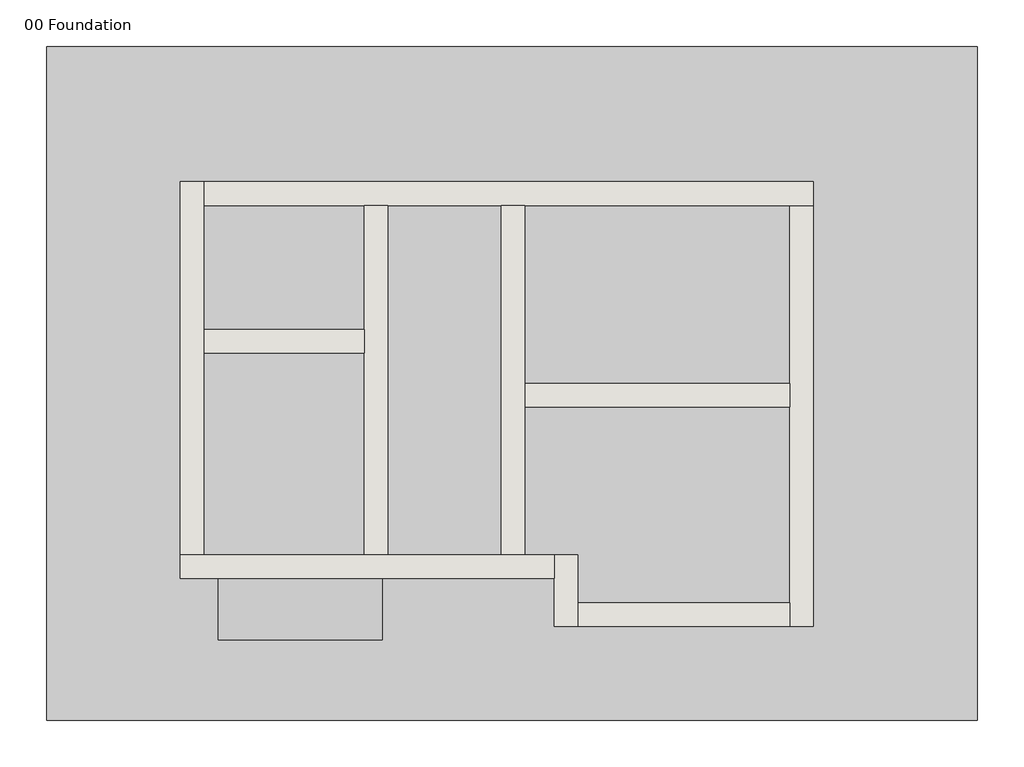
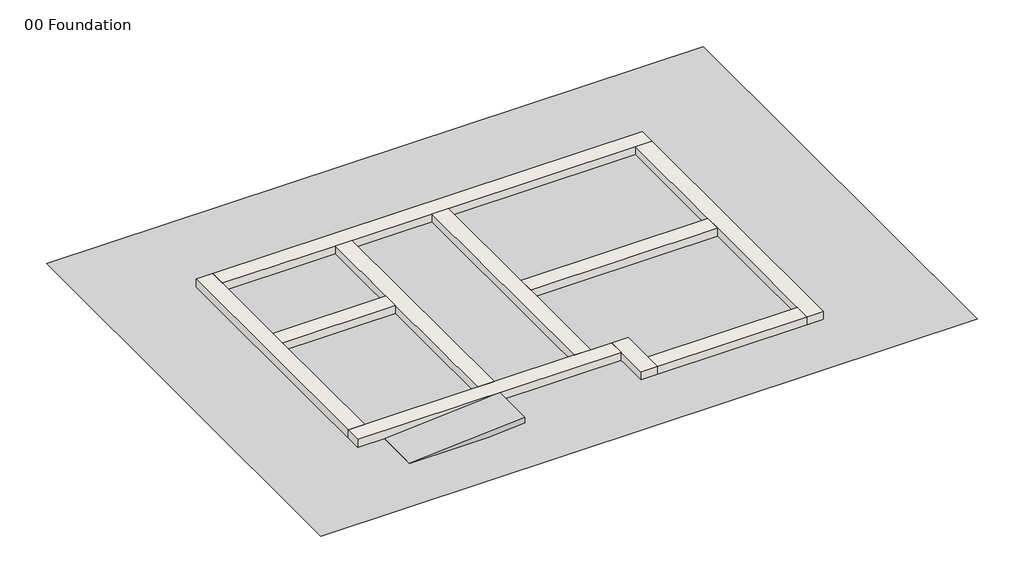
# One storey: 10 footings, 10 walls, 1 proxy, 1 ramp.
"""IFC4 building model written with IfcOpenShell, lengths in millimetres."""

import ifcopenshell
import ifcopenshell.guid

model = None  # the IFC model being written
_history = None  # IfcOwnerHistory: only IFC2X3 demands one
_inside = {}  # id of a spatial element -> (the spatial element, [elements in it])
_under = {}  # id of a project, library or spatial element -> (it, [spatial elements below it])
_declared = {}  # id of a project -> (the project, [libraries it declares])
_typed = {}  # id of a type object -> (the type object, [elements of that type])
_made_of = {}  # id of a material, layer set ... -> (it, [elements and type objects made of it])


def new_model(schema):
    """Start an empty IFC model of exactly this schema.

    Asked for "IFC4X3", IfcOpenShell would pick the latest addendum, in which some entities
    have other attributes; the version numbers below select the first issue.
    IFC2X3 requires an IfcOwnerHistory on every rooted entity: one is made here for all.
    """
    global model, _history
    if schema == "IFC4X3":
        model = ifcopenshell.file(schema_version=(4, 3, 0, 0))
    else:
        model = ifcopenshell.file(schema=schema)
    _inside.clear()
    _under.clear()
    _declared.clear()
    _typed.clear()
    _made_of.clear()
    _history = None
    if model.schema == "IFC2X3":
        org = make("IfcOrganization", Name="unknown")
        user = make(
            "IfcPersonAndOrganization",
            ThePerson=make("IfcPerson", FamilyName="unknown"),
            TheOrganization=org,
        )
        app = make(
            "IfcApplication",
            ApplicationDeveloper=org,
            Version="unknown",
            ApplicationFullName="unknown",
            ApplicationIdentifier="unknown",
        )
        _history = make(
            "IfcOwnerHistory",
            OwningUser=user,
            OwningApplication=app,
            ChangeAction="ADDED",
            CreationDate=0,
        )
    return model


def make(cls, **values):
    """One entity of the class cls with the attributes given. An attribute that is None is left unset."""
    return model.create_entity(
        cls, **{name: value for name, value in values.items() if value is not None}
    )


def rooted(cls, **values):
    """An entity with a GlobalId (a new one), such as an element, a storey or a relation."""
    return make(cls, GlobalId=ifcopenshell.guid.new(), OwnerHistory=_history, **values)


def si_unit(unit_type, name, prefix=None):
    """IfcSIUnit, for example si_unit("LENGTHUNIT", "METRE", prefix="MILLI")."""
    return make("IfcSIUnit", UnitType=unit_type, Prefix=prefix, Name=name)


def assignment(units):
    """IfcUnitAssignment: the units of a project."""
    return None if units is None else make("IfcUnitAssignment", Units=units)


def point(xyz):
    """IfcCartesianPoint."""
    return None if xyz is None else make("IfcCartesianPoint", Coordinates=xyz)


def direction(xyz):
    """IfcDirection."""
    return None if xyz is None else make("IfcDirection", DirectionRatios=xyz)


def frame(location, z_axis=None, x_axis=None):
    """IfcAxis2Placement3D, a coordinate frame: its origin and axes. An axis left out is left unset."""
    return make(
        "IfcAxis2Placement3D",
        Location=point(location),
        Axis=direction(z_axis),
        RefDirection=direction(x_axis),
    )


def origin():
    """The frame at (0, 0, 0) with its axes left unset."""
    return frame((0.0, 0.0, 0.0))


def place(relative_to, where):
    """IfcLocalPlacement: puts the frame where relative to a parent placement (None: the world)."""
    return make(
        "IfcLocalPlacement", PlacementRelTo=relative_to, RelativePlacement=where
    )


def context(
    kind, dimensions, precision=None, world=None, true_north=None, identifier=None
):
    """IfcGeometricRepresentationContext, for example the 3D "Model" context."""
    return make(
        "IfcGeometricRepresentationContext",
        ContextIdentifier=identifier,
        ContextType=kind,
        CoordinateSpaceDimension=dimensions,
        Precision=precision,
        WorldCoordinateSystem=world,
        TrueNorth=true_north,
    )


def project(units=None, contexts=None):
    """IfcProject with its units and contexts."""
    return rooted(
        "IfcProject",
        Name="project",
        RepresentationContexts=contexts,
        UnitsInContext=assignment(units),
    )


def spatial(cls, under=None, at=None, **own):
    """A site, building, storey or space (cls), placed at a placement, below another one or the project."""
    s = rooted(cls, ObjectPlacement=at, **own)
    if under is not None:
        _under.setdefault(under.id(), (under, []))[1].append(s)
    return s


def polyline(points):
    """IfcPolyline through the points."""
    return make("IfcPolyline", Points=[point(p) for p in points])


def point_list(points):
    """IfcCartesianPointList2D or 3D."""
    cls = (
        "IfcCartesianPointList2D" if len(points[0]) == 2 else "IfcCartesianPointList3D"
    )
    return make(cls, CoordList=points)


def outline(outer, holes=None, kind="AREA"):
    """IfcArbitraryClosedProfileDef: a profile drawn as a closed curve; with holes, ...WithVoids."""
    if holes is None:
        return make("IfcArbitraryClosedProfileDef", ProfileType=kind, OuterCurve=outer)
    return make(
        "IfcArbitraryProfileDefWithVoids",
        ProfileType=kind,
        OuterCurve=outer,
        InnerCurves=holes,
    )


def extrude(swept, where, along, depth):
    """IfcExtrudedAreaSolid: the profile swept, set in the frame where, extruded along a direction by depth."""
    return make(
        "IfcExtrudedAreaSolid",
        SweptArea=swept,
        Position=where,
        ExtrudedDirection=direction(along),
        Depth=depth,
    )


def faces_of(points, faces, orient=None, outer=None):
    """IfcFace entities. A face is a list of loops; a loop is a list of indices into points, from 0.

    orient and outer hold one flag for each loop. By default every Orientation is true, the
    first loop of a face is its IfcFaceOuterBound and the others are IfcFaceBound.
    """
    made = []
    for i, loops in enumerate(faces):
        bounds = []
        for j, loop in enumerate(loops):
            is_outer = j == 0 if outer is None else outer[i][j]
            bounds.append(
                make(
                    "IfcFaceOuterBound" if is_outer else "IfcFaceBound",
                    Bound=make("IfcPolyLoop", Polygon=[points[k] for k in loop]),
                    Orientation=True if orient is None else orient[i][j],
                )
            )
        made.append(make("IfcFace", Bounds=bounds))
    return made


def faceted_brep(points, faces, orient=None, outer=None, voids=None):
    """IfcFacetedBrep: a solid bounded by flat faces; with voids (closed shells), ...WithVoids."""
    shared = [point(p) for p in points]
    hull = make("IfcClosedShell", CfsFaces=faces_of(shared, faces, orient, outer))
    if voids is None:
        return make("IfcFacetedBrep", Outer=hull)
    return make(
        "IfcFacetedBrepWithVoids",
        Outer=hull,
        Voids=[
            make(cls, CfsFaces=faces_of(shared, fs, o, b)) for cls, fs, o, b in voids
        ],
    )


def triangles(points, corners, closed=None, point_numbers=None):
    """IfcTriangulatedFaceSet: each triangle names its three corners, points numbered from 1."""
    return make(
        "IfcTriangulatedFaceSet",
        Coordinates=point_list(points),
        Closed=closed,
        CoordIndex=corners,
        PnIndex=point_numbers,
    )


def shape(context_of_items, identifier, shape_type, items):
    """IfcShapeRepresentation: the items that make up one representation, for example the "Body"."""
    return make(
        "IfcShapeRepresentation",
        ContextOfItems=context_of_items,
        RepresentationIdentifier=identifier,
        RepresentationType=shape_type,
        Items=items,
    )


def source(mapping_origin, context_of_items, identifier, shape_type, items):
    """IfcRepresentationMap: a shape defined once, which mapped items show again and again."""
    return make(
        "IfcRepresentationMap",
        MappingOrigin=mapping_origin,
        MappedRepresentation=shape(context_of_items, identifier, shape_type, items),
    )


def transform(
    local_origin,
    x_axis=None,
    y_axis=None,
    z_axis=None,
    scale=None,
    scale2=None,
    scale3=None,
    uniform=True,
):
    """IfcCartesianTransformationOperator3D, or its non-uniform kind. x_axis, y_axis, z_axis: its Axis1, 2, 3."""
    if uniform:
        return make(
            "IfcCartesianTransformationOperator3D",
            Axis1=direction(x_axis),
            Axis2=direction(y_axis),
            LocalOrigin=point(local_origin),
            Scale=scale,
            Axis3=direction(z_axis),
        )
    return make(
        "IfcCartesianTransformationOperator3DnonUniform",
        Axis1=direction(x_axis),
        Axis2=direction(y_axis),
        LocalOrigin=point(local_origin),
        Scale=scale,
        Axis3=direction(z_axis),
        Scale2=scale2,
        Scale3=scale3,
    )


def mapped(mapping_source, mapping_target):
    """IfcMappedItem: shows the shape of a source again, moved by a transform."""
    return make(
        "IfcMappedItem", MappingSource=mapping_source, MappingTarget=mapping_target
    )


def made_of(thing, what):
    """Note that an element or type object is made of a material, layer set ...; save() writes the relation."""
    if what is not None:
        _made_of.setdefault(what.id(), (what, []))[1].append(thing)
    return thing


def element(
    cls,
    number,
    at=None,
    inside=None,
    cuts=None,
    type_object=None,
    material=None,
    context=None,
    identifier="Body",
    shape_type=None,
    held_by="IfcProductDefinitionShape",
    body=None,
    shapes=None,
    **own,
):
    """One element of the class cls, such as IfcWall. Its Tag is "e" and its number.

    at: its placement. inside: the storey or other place that contains it. cuts: it is an
    opening in that element (IfcRelVoidsElement). A single representation is given by context,
    identifier, shape_type and body (its items); several are given by shapes. held_by: the class
    of the entity that holds the representations. save() writes the other relations.
    """
    e = rooted(cls, Tag="e%d" % number, ObjectPlacement=at, **own)
    if body is not None:
        shapes = [shape(context, identifier, shape_type, body)]
    if shapes is not None:
        e.Representation = make(held_by, Representations=shapes)
    if inside is not None:
        _inside.setdefault(inside.id(), (inside, []))[1].append(e)
    if cuts is not None:
        rooted(
            "IfcRelVoidsElement", RelatingBuildingElement=cuts, RelatedOpeningElement=e
        )
    if type_object is not None:
        _typed.setdefault(type_object.id(), (type_object, []))[1].append(e)
    return made_of(e, material)


def aggregate(whole, parts):
    """IfcRelAggregates: a whole, such as a stair, and the parts it consists of."""
    return rooted("IfcRelAggregates", RelatingObject=whole, RelatedObjects=parts)


def save(model, path):
    """Write the relations noted so far, then the file.

    IfcRelAggregates (storeys below a building ...), IfcRelContainedInSpatialStructure (elements
    in a storey), IfcRelDefinesByType, IfcRelAssociatesMaterial and IfcRelDeclares: one each for
    every whole, place, type object, material and project.
    """
    for whole, parts in _under.values():
        aggregate(whole, parts)
    for where, things in _inside.values():
        rooted(
            "IfcRelContainedInSpatialStructure",
            RelatedElements=things,
            RelatingStructure=where,
        )
    for kind, things in _typed.values():
        rooted("IfcRelDefinesByType", RelatedObjects=things, RelatingType=kind)
    for what, things in _made_of.values():
        rooted("IfcRelAssociatesMaterial", RelatedObjects=things, RelatingMaterial=what)
    for by, libraries in _declared.values():
        rooted("IfcRelDeclares", RelatingContext=by, RelatedDefinitions=libraries)
    model.write(path)


def ramp_1_ce501800(model_context):
    return source(origin(), model_context, "Body", "SweptSolid", [
        extrude(outline(polyline([(0.0, -7500.2064028), (-225.0, -10560.2064028), (-375.4049465, -10560.2064028), (-150.4049465, -7500.2064028), (0.0, -7500.2064028)])), frame((0.0, -1636.162817, 0.0), z_axis=(0.0, 1.0, 0.0), x_axis=(0.0, 0.0, 1.0)), (0.0, 0.0, 1.0), 1200.0),
    ])


model = new_model("IFC4")

# Units and contexts
model_context = context("Model", 3, world=origin())
ifc_project = project(units=[si_unit("LENGTHUNIT", "METRE", prefix="MILLI")], contexts=[model_context])

# Site, building, storey
site = spatial("IfcSite", under=ifc_project)
building = spatial("IfcBuilding", under=site)
storey = spatial("IfcBuildingStorey", under=building, Name="00 Foundation", Elevation=-900.0)

# Proxy
placement = place(None, origin())
element("IfcBuildingElementProxy", 1, Name="Building Element Proxy", at=placement, inside=storey, context=model_context, shape_type="Tessellation", body=[
    triangles([(-13772.2558685, 9461.3562103, -225.0000017), (3627.7439735, 9461.3562103, -225.0000017), (3627.7439735, -3138.6435951, -225.0000017), (-13772.2558685, -3138.6435951, -225.0000017)], [[1, 4, 2], [3, 2, 4]], closed=False),
])

# Footings
element("IfcFooting", 2, ObjectType="Wall Foundation Domestic 910", at=placement, inside=storey, context=model_context, shape_type="Brep", body=[
    faceted_brep([(-10595.3997381, -720.6350684, -900.0), (-10595.3997381, 189.3649316, -900.0), (-10595.3997381, 3496.6149316, -900.0), (-10595.3997381, 4406.6149316, -900.0), (-10595.3997381, 6255.1149316, -900.0), (-10595.3997381, 7165.1149316, -900.0), (-11505.3997381, 7165.1149316, -900.0), (-11505.3997381, -720.6350684, -900.0), (-11505.3997381, -720.6350684, -1250.0), (-11505.3997381, 7165.1149316, -1250.0), (-10595.3997381, -720.6350684, -1250.0), (-10595.3997381, 7165.1149316, -1250.0), (-10595.3997381, 6255.1149316, -1250.0), (-10595.3997381, 4406.6149316, -1250.0), (-10595.3997381, 3496.6149316, -1250.0), (-10595.3997381, 189.3649316, -1250.0)], [[[0, 1, 2, 3, 4, 5, 6, 7]], [[8, 7, 6, 9]], [[10, 8, 9, 11, 12, 13, 14, 15]], [[0, 10, 15, 14, 13, 12, 11, 5, 4, 3, 2, 1]], [[6, 5, 11, 9]], [[0, 7, 8, 10]]]),
])
element("IfcFooting", 3, ObjectType="Wall Foundation Domestic 910", at=placement, inside=storey, context=model_context, shape_type="Brep", body=[
    faceted_brep([(792.3502619, 6255.1149316, -900.0), (792.3502619, 7165.1149316, -900.0), (-10595.3997381, 7165.1149316, -900.0), (-10595.3997381, 6255.1149316, -900.0), (-8069.2747381, 6255.1149316, -900.0), (-7159.2747381, 6255.1149316, -900.0), (-5512.2747381, 6255.1149316, -900.0), (-4602.2747381, 6255.1149316, -900.0), (-117.6497381, 6255.1149316, -900.0), (792.3502619, 7165.1149316, -1250.0), (-10595.3997381, 7165.1149316, -1250.0), (792.3502619, 6255.1149316, -1250.0), (-117.6497381, 6255.1149316, -1250.0), (-4602.2747381, 6255.1149316, -1250.0), (-5512.2747381, 6255.1149316, -1250.0), (-7159.2747381, 6255.1149316, -1250.0), (-8069.2747381, 6255.1149316, -1250.0), (-10595.3997381, 6255.1149316, -1250.0)], [[[0, 1, 2, 3, 4, 5, 6, 7, 8]], [[1, 9, 10, 2]], [[9, 11, 12, 13, 14, 15, 16, 17, 10]], [[11, 0, 8, 7, 6, 5, 4, 3, 17, 16, 15, 14, 13, 12]], [[3, 2, 10, 17]], [[1, 0, 11, 9]]]),
])
element("IfcFooting", 4, ObjectType="Wall Foundation Domestic 910", at=placement, inside=storey, context=model_context, shape_type="Brep", body=[
    faceted_brep([(-10595.3997381, 3496.6149316, -900.0), (-8069.2747381, 3496.6149316, -900.0), (-7159.2747381, 3496.6149316, -900.0), (-7159.2747381, 4406.6149316, -900.0), (-8069.2747381, 4406.6149316, -900.0), (-10595.3997381, 4406.6149316, -900.0), (-10595.3997381, 4406.6149316, -1250.0), (-7159.2747381, 4406.6149316, -1250.0), (-8069.2747381, 4406.6149316, -1250.0), (-10595.3997381, 3496.6149316, -1250.0), (-7159.2747381, 3496.6149316, -1250.0), (-8069.2747381, 3496.6149316, -1250.0)], [[[0, 1, 2, 3, 4, 5]], [[6, 5, 4, 3, 7, 8]], [[9, 6, 8, 7, 10, 11]], [[0, 9, 11, 10, 2, 1]], [[0, 5, 6, 9]], [[3, 2, 10, 7]]]),
])
element("IfcFooting", 5, ObjectType="Wall Foundation Domestic 910", at=placement, inside=storey, context=model_context, shape_type="SweptSolid", body=[
    extrude(outline(polyline([(-8069.2747381, 6255.1149316), (-7159.2747381, 6255.1149316), (-7159.2747381, 4406.6149316), (-8069.2747381, 4406.6149316), (-8069.2747381, 6255.1149316)])), frame((0.0, 0.0, -1250.0), z_axis=(0.0, 0.0, 1.0), x_axis=(1.0, 0.0, 0.0)), (0.0, 0.0, 1.0), 350.0),
    extrude(outline(polyline([(-7159.2747381, 189.3649316), (-8069.2747381, 189.3649316), (-8069.2747381, 3496.6149316), (-7159.2747381, 3496.6149316), (-7159.2747381, 189.3649316)])), frame((0.0, 0.0, -1250.0), z_axis=(0.0, 0.0, 1.0), x_axis=(1.0, 0.0, 0.0)), (0.0, 0.0, 1.0), 350.0),
])
element("IfcFooting", 6, ObjectType="Wall Foundation Domestic 910", at=placement, inside=storey, context=model_context, shape_type="Brep", body=[
    faceted_brep([(-5512.2747381, 6255.1149316, -900.0), (-5512.2747381, 189.3649316, -900.0), (-4602.2747381, 189.3649316, -900.0), (-4602.2747381, 2480.3649316, -900.0), (-4602.2747381, 3390.3649316, -900.0), (-4602.2747381, 6255.1149316, -900.0), (-4602.2747381, 6255.1149316, -1250.0), (-4602.2747381, 189.3649316, -1250.0), (-4602.2747381, 2480.3649316, -1250.0), (-4602.2747381, 3390.3649316, -1250.0), (-5512.2747381, 6255.1149316, -1250.0), (-5512.2747381, 189.3649316, -1250.0)], [[[0, 1, 2, 3, 4, 5]], [[6, 5, 4, 3, 2, 7, 8, 9]], [[10, 6, 9, 8, 7, 11]], [[0, 10, 11, 1]], [[0, 5, 6, 10]], [[2, 1, 11, 7]]]),
])
element("IfcFooting", 7, ObjectType="Wall Foundation Domestic 910", at=placement, inside=storey, context=model_context, shape_type="SweptSolid", body=[
    extrude(outline(polyline([(-117.6497381, 3390.3649316), (-117.6497381, 2480.3649316), (-4602.2747381, 2480.3649316), (-4602.2747381, 3390.3649316), (-117.6497381, 3390.3649316)])), frame((0.0, 0.0, -1250.0), z_axis=(0.0, 0.0, 1.0), x_axis=(1.0, 0.0, 0.0)), (0.0, 0.0, 1.0), 350.0),
])
element("IfcFooting", 8, ObjectType="Wall Foundation Domestic 910", at=placement, inside=storey, context=model_context, shape_type="Brep", body=[
    faceted_brep([(-117.6497381, -1620.6350684, -900.0), (792.3502619, -1620.6350684, -900.0), (792.3502619, 6255.1149316, -900.0), (-117.6497381, 6255.1149316, -900.0), (-117.6497381, 3390.3649316, -900.0), (-117.6497381, 2480.3649316, -900.0), (-117.6497381, -710.6350684, -900.0), (792.3502619, -1620.6350684, -1250.0), (792.3502619, 6255.1149316, -1250.0), (-117.6497381, -1620.6350684, -1250.0), (-117.6497381, -710.6350684, -1250.0), (-117.6497381, 2480.3649316, -1250.0), (-117.6497381, 3390.3649316, -1250.0), (-117.6497381, 6255.1149316, -1250.0)], [[[0, 1, 2, 3, 4, 5, 6]], [[1, 7, 8, 2]], [[7, 9, 10, 11, 12, 13, 8]], [[9, 0, 6, 5, 4, 3, 13, 12, 11, 10]], [[3, 2, 8, 13]], [[1, 0, 9, 7]]]),
])
element("IfcFooting", 9, ObjectType="Wall Foundation Domestic 910", at=placement, inside=storey, context=model_context, shape_type="Brep", body=[
    faceted_brep([(-3609.7747381, -720.6350684, -900.0), (-3609.7747381, -710.6350684, -900.0), (-3609.7747381, 189.3649316, -900.0), (-4602.2747381, 189.3649316, -900.0), (-5512.2747381, 189.3649316, -900.0), (-7159.2747381, 189.3649316, -900.0), (-8069.2747381, 189.3649316, -900.0), (-10595.3997381, 189.3649316, -900.0), (-10595.3997381, -720.6350684, -900.0), (-4519.7747381, -720.6350684, -900.0), (-3609.7747381, -720.6350684, -1250.0), (-10595.3997381, -720.6350684, -1250.0), (-4519.7747381, -720.6350684, -1250.0), (-3609.7747381, 189.3649316, -1250.0), (-3609.7747381, -710.6350684, -1250.0), (-10595.3997381, 189.3649316, -1250.0), (-8069.2747381, 189.3649316, -1250.0), (-7159.2747381, 189.3649316, -1250.0), (-5512.2747381, 189.3649316, -1250.0), (-4602.2747381, 189.3649316, -1250.0)], [[[0, 1, 2, 3, 4, 5, 6, 7, 8, 9]], [[10, 0, 9, 8, 11, 12]], [[13, 14, 10, 12, 11, 15, 16, 17, 18, 19]], [[2, 13, 19, 18, 17, 16, 15, 7, 6, 5, 4, 3]], [[8, 7, 15, 11]], [[2, 1, 0, 10, 14, 13]]]),
])
element("IfcFooting", 10, ObjectType="Wall Foundation Domestic 910", at=placement, inside=storey, context=model_context, shape_type="SweptSolid", body=[
    extrude(outline(polyline([(-3609.7747381, -1620.6350684), (-4519.7747381, -1620.6350684), (-4519.7747381, -720.6350684), (-3609.7747381, -720.6350684), (-3609.7747381, -1620.6350684)])), frame((0.0, 0.0, -1250.0), z_axis=(0.0, 0.0, 1.0), x_axis=(1.0, 0.0, 0.0)), (0.0, 0.0, 1.0), 350.0),
])
element("IfcFooting", 11, ObjectType="Wall Foundation Domestic 910", at=placement, inside=storey, context=model_context, shape_type="Brep", body=[
    faceted_brep([(-117.6497381, -1620.6350684, -900.0), (-117.6497381, -710.6350684, -900.0), (-3609.7747381, -710.6350684, -900.0), (-3609.7747381, -720.6350684, -900.0), (-3609.7747381, -1620.6350684, -900.0), (-117.6497381, -1620.6350684, -1250.0), (-3609.7747381, -1620.6350684, -1250.0), (-117.6497381, -710.6350684, -1250.0), (-3609.7747381, -720.6350684, -1250.0), (-3609.7747381, -710.6350684, -1250.0)], [[[0, 1, 2, 3, 4]], [[5, 0, 4, 6]], [[7, 5, 6, 8, 9]], [[1, 7, 9, 2]], [[1, 0, 5, 7]], [[2, 9, 8, 6, 4, 3]]]),
])

# Ramp
ramp_1_shape = ramp_1_ce501800(model_context)
element("IfcRamp", 12, ObjectType="Ramp 1", at=placement, inside=storey, context=model_context, shape_type="MappedRepresentation", body=[
    mapped(ramp_1_shape, transform((0.0, 0.0, 0.0), x_axis=(1.0, 0.0, 0.0), y_axis=(0.0, 1.0, 0.0), z_axis=(0.0, 0.0, 1.0))),
])

# Walls
element("IfcWall", 13, ObjectType="L4_Wall-Fnd_440DBlk (Trench Blockwork)", at=placement, inside=storey, context=model_context, shape_type="Brep", body=[
    faceted_brep([(-10830.3997381, -45.6350684, -900.0), (-10830.3997381, 3731.6149316, -900.0), (-10830.3997381, 4171.6149316, -900.0), (-10830.3997381, 6490.1149316, -900.0), (-10830.3997381, 6930.1149316, -900.0), (-10830.3997381, 6930.1149316, 0.0), (-10830.3997381, 6490.1149316, 0.0), (-10830.3997381, 4171.6149316, 0.0), (-10830.3997381, 3731.6149316, 0.0), (-10830.3997381, -45.6350684, 0.0), (-11270.3997381, -45.6350684, -900.0), (-11270.3997381, -45.6350684, 0.0), (-11270.3997381, 6930.1149316, 0.0), (-11270.3997381, 6930.1149316, -900.0)], [[[0, 1, 2, 3, 4, 5, 6, 7, 8, 9]], [[10, 11, 12, 13]], [[4, 3, 2, 1, 0, 10, 13]], [[9, 8, 7, 6, 5, 12, 11]], [[5, 4, 13, 12]], [[0, 9, 11, 10]]]),
])
element("IfcWall", 14, ObjectType="L4_Wall-Fnd_440DBlk (Trench Blockwork)", at=placement, inside=storey, context=model_context, shape_type="Brep", body=[
    faceted_brep([(-10830.3997381, 6490.1149316, -900.0), (-7834.2747381, 6490.1149316, -900.0), (-7394.2747381, 6490.1149316, -900.0), (-5277.2747381, 6490.1149316, -900.0), (-4837.2747381, 6490.1149316, -900.0), (117.3502619, 6490.1149316, -900.0), (557.3502619, 6490.1149316, -900.0), (557.3502619, 6490.1149316, 0.0), (117.3502619, 6490.1149316, 0.0), (-4837.2747381, 6490.1149316, 0.0), (-5277.2747381, 6490.1149316, 0.0), (-7394.2747381, 6490.1149316, 0.0), (-7834.2747381, 6490.1149316, 0.0), (-10830.3997381, 6490.1149316, 0.0), (-10830.3997381, 6930.1149316, -900.0), (-10830.3997381, 6930.1149316, 0.0), (557.3502619, 6930.1149316, 0.0), (557.3502619, 6930.1149316, -900.0)], [[[0, 1, 2, 3, 4, 5, 6, 7, 8, 9, 10, 11, 12, 13]], [[14, 15, 16, 17]], [[6, 5, 4, 3, 2, 1, 0, 14, 17]], [[13, 12, 11, 10, 9, 8, 7, 16, 15]], [[0, 13, 15, 14]], [[7, 6, 17, 16]]]),
])
element("IfcWall", 15, ObjectType="L4_Wall-Fnd_440DBlk (Trench Blockwork)", at=placement, inside=storey, context=model_context, shape_type="Brep", body=[
    faceted_brep([(117.3502619, 6490.1149316, -900.0), (117.3502619, 3155.3649316, -900.0), (117.3502619, 2715.3649316, -900.0), (117.3502619, -945.6350684, -900.0), (117.3502619, -1385.6350684, -900.0), (117.3502619, -1385.6350684, 0.0), (117.3502619, -945.6350684, 0.0), (117.3502619, 2715.3649316, 0.0), (117.3502619, 3155.3649316, 0.0), (117.3502619, 6490.1149316, 0.0), (557.3502619, 6490.1149316, -900.0), (557.3502619, 6490.1149316, 0.0), (557.3502619, -1385.6350684, 0.0), (557.3502619, -1385.6350684, -900.0)], [[[0, 1, 2, 3, 4, 5, 6, 7, 8, 9]], [[10, 11, 12, 13]], [[4, 3, 2, 1, 0, 10, 13]], [[9, 8, 7, 6, 5, 12, 11]], [[5, 4, 13, 12]], [[0, 9, 11, 10]]]),
])
element("IfcWall", 16, ObjectType="L4_Wall-Fnd_440DBlk (Trench Blockwork)", at=placement, inside=storey, context=model_context, shape_type="Brep", body=[
    faceted_brep([(-4284.7747381, -45.6350684, -900.0), (-4837.2747381, -45.6350684, -900.0), (-5277.2747381, -45.6350684, -900.0), (-7394.2747381, -45.6350684, -900.0), (-7834.2747381, -45.6350684, -900.0), (-10830.3997381, -45.6350684, -900.0), (-11270.3997381, -45.6350684, -900.0), (-11270.3997381, -45.6350684, 0.0), (-10830.3997381, -45.6350684, 0.0), (-7834.2747381, -45.6350684, 0.0), (-7394.2747381, -45.6350684, 0.0), (-5277.2747381, -45.6350684, 0.0), (-4837.2747381, -45.6350684, 0.0), (-4284.7747381, -45.6350684, 0.0), (-4284.7747381, -485.6350684, -900.0), (-4284.7747381, -485.6350684, 0.0), (-11270.3997381, -485.6350684, 0.0), (-11270.3997381, -485.6350684, -900.0)], [[[0, 1, 2, 3, 4, 5, 6, 7, 8, 9, 10, 11, 12, 13]], [[14, 15, 16, 17]], [[6, 5, 4, 3, 2, 1, 0, 14, 17]], [[13, 12, 11, 10, 9, 8, 7, 16, 15]], [[7, 6, 17, 16]], [[0, 13, 15, 14]]]),
])
element("IfcWall", 17, ObjectType="L4_Wall-Fnd_440DBlk (Trench Blockwork)", at=placement, inside=storey, context=model_context, shape_type="SweptSolid", body=[
    extrude(outline(polyline([(-3844.7747381, -945.6350684), (117.3502619, -945.6350684), (117.3502619, -1385.6350684), (-3844.7747381, -1385.6350684), (-3844.7747381, -945.6350684)])), frame((0.0, 0.0, -900.0), z_axis=(0.0, 0.0, 1.0), x_axis=(1.0, 0.0, 0.0)), (0.0, 0.0, 1.0), 900.0),
])
element("IfcWall", 18, ObjectType="L4_Wall-Fnd_440DBlk (Trench Blockwork)", at=placement, inside=storey, context=model_context, shape_type="Brep", body=[
    faceted_brep([(-3844.7747381, -1385.6350684, -900.0), (-3844.7747381, -945.6350684, -900.0), (-3844.7747381, -45.6350684, -900.0), (-3844.7747381, -45.6350684, 0.0), (-3844.7747381, -945.6350684, 0.0), (-3844.7747381, -1385.6350684, 0.0), (-4284.7747381, -1385.6350684, -900.0), (-4284.7747381, -1385.6350684, 0.0), (-4284.7747381, -485.6350684, 0.0), (-4284.7747381, -45.6350684, 0.0), (-4284.7747381, -45.6350684, -900.0), (-4284.7747381, -485.6350684, -900.0)], [[[0, 1, 2, 3, 4, 5]], [[6, 7, 8, 9, 10, 11]], [[2, 1, 0, 6, 11, 10]], [[5, 4, 3, 9, 8, 7]], [[3, 2, 10, 9]], [[0, 5, 7, 6]]]),
])
element("IfcWall", 19, ObjectType="L4_Wall-Fnd_440DBlk (Trench Blockwork)", at=placement, inside=storey, context=model_context, shape_type="SweptSolid", body=[
    extrude(outline(polyline([(-7834.2747381, 3731.6149316), (-10830.3997381, 3731.6149316), (-10830.3997381, 4171.6149316), (-7834.2747381, 4171.6149316), (-7834.2747381, 3731.6149316)])), frame((0.0, 0.0, -900.0), z_axis=(0.0, 0.0, 1.0), x_axis=(1.0, 0.0, 0.0)), (0.0, 0.0, 1.0), 900.0),
])
element("IfcWall", 20, ObjectType="L4_Wall-Fnd_440DBlk (Trench Blockwork)", at=placement, inside=storey, context=model_context, shape_type="Brep", body=[
    faceted_brep([(-7394.2747381, -45.6350684, -900.0), (-7394.2747381, 6490.1149316, -900.0), (-7394.2747381, 6490.1149316, 0.0), (-7394.2747381, -45.6350684, 0.0), (-7834.2747381, -45.6350684, -900.0), (-7834.2747381, -45.6350684, 0.0), (-7834.2747381, 3731.6149316, 0.0), (-7834.2747381, 4171.6149316, 0.0), (-7834.2747381, 6490.1149316, 0.0), (-7834.2747381, 6490.1149316, -900.0), (-7834.2747381, 4171.6149316, -900.0), (-7834.2747381, 3731.6149316, -900.0)], [[[0, 1, 2, 3]], [[4, 5, 6, 7, 8, 9, 10, 11]], [[1, 0, 4, 11, 10, 9]], [[3, 2, 8, 7, 6, 5]], [[2, 1, 9, 8]], [[0, 3, 5, 4]]]),
])
element("IfcWall", 21, ObjectType="L4_Wall-Fnd_440DBlk (Trench Blockwork)", at=placement, inside=storey, context=model_context, shape_type="Brep", body=[
    faceted_brep([(-5277.2747381, 6490.1149316, -900.0), (-5277.2747381, -45.6350684, -900.0), (-5277.2747381, -45.6350684, 0.0), (-5277.2747381, 6490.1149316, 0.0), (-4837.2747381, 6490.1149316, -900.0), (-4837.2747381, 6490.1149316, 0.0), (-4837.2747381, 3155.3649316, 0.0), (-4837.2747381, 2715.3649316, 0.0), (-4837.2747381, -45.6350684, 0.0), (-4837.2747381, -45.6350684, -900.0), (-4837.2747381, 2715.3649316, -900.0), (-4837.2747381, 3155.3649316, -900.0)], [[[0, 1, 2, 3]], [[4, 5, 6, 7, 8, 9, 10, 11]], [[1, 0, 4, 11, 10, 9]], [[3, 2, 8, 7, 6, 5]], [[0, 3, 5, 4]], [[2, 1, 9, 8]]]),
])
element("IfcWall", 22, ObjectType="L4_Wall-Fnd_440DBlk (Trench Blockwork)", at=placement, inside=storey, context=model_context, shape_type="SweptSolid", body=[
    extrude(outline(polyline([(117.3502619, 2715.3649316), (-4837.2747381, 2715.3649316), (-4837.2747381, 3155.3649316), (117.3502619, 3155.3649316), (117.3502619, 2715.3649316)])), frame((0.0, 0.0, -900.0), z_axis=(0.0, 0.0, 1.0), x_axis=(1.0, 0.0, 0.0)), (0.0, 0.0, 1.0), 900.0),
])

save(model, "model.ifc")

# Revit data of these elements
# Project information
#   Document_Suitability_Code = "A1"
#   Document_Suitability_Description = "Coordination"
#   Project Issue Date = "22-Feb-23"
#   Project Status = "Project Status"
#   Client Name = "Revit Project"
#   Project Address = "Enter address here"
#   Project Name = "Two Storey House"
#   Project Number = "RARC01"
# Type "Ramp 1"
#   built-in parameter 1008304 = 0.492126 (stored number, unit not read)
#   built-in parameter 1008303 = 39.3701 (stored number, unit not read)
#   built-in parameter 1008301 = 12 (stored number, unit not read)
#   Function = 1
#   built-in parameter 1008308 = Concrete, Cast In Situ
# Type "L4_Wall-Fnd_440DBlk (Trench Blockwork)"
#   Keynote = "F10"
#   Layers, outside or top first: 440 mm "Concrete Masonry Units 440" (function 1)
# Element 1 (IfcBuildingElementProxy)
#   Material = Asphalt, Pavement
#   Phase Created = New Construction
# Elements 2, 3, 4, 5, 6, 7, 8, 9, 10, 11 (IfcFooting, "Wall Foundation Domestic 910")
#   Comments = ""
#   Phase Created = New Construction
#   Materials on its faces: "Concrete, Cast In Situ"
# Element 12 (IfcRamp, "Ramp 1")
#   built-in parameter 1007275 = "DN"
#   built-in parameter 1007272 = "UP"
#   built-in parameter 1007218 = -0.738189 (stored number, unit not read)
#   Width = 1200 mm
#   built-in parameter 1007276 = 1
#   built-in parameter 1007274 = 1
#   built-in parameter 1007273 = 1
#   built-in parameter 1007271 = 1
#   Phase Created = New Construction
#   Materials on its faces: "Concrete, Cast In Situ"
# Elements 13, 14, 15, 16, 17, 18, 19, 20, 21, 22 (IfcWall, "L4_Wall-Fnd_440DBlk (Trench Blockwork)")
#   Top Offset = 0 mm
#   Base Offset = 0 mm
#   wall height = 900 mm
#   Phase Created = New Construction
#   Base Constraint = 00 Foundation
#   Top Constraint = 00 Ground Floor
#   Materials on its faces: "Concrete Masonry Units 440"
# Materials
#   "Concrete, Cast In Situ": class "Concrete", colour RGB 192 192 192, transparency 0, Keynote = "F30/110", Description = "physical material", Cost = 0
#   "Concrete Masonry Units 440": class "Masonry", colour RGB 152 154 138, transparency 0, Keynote = "F10/350", Description = "Concrete masonry units", Cost = 0
#   "Asphalt, Pavement": class "Generic", colour RGB 192 192 192, transparency 0, Description = "Asphalt or tarmac paving", Cost = 0
